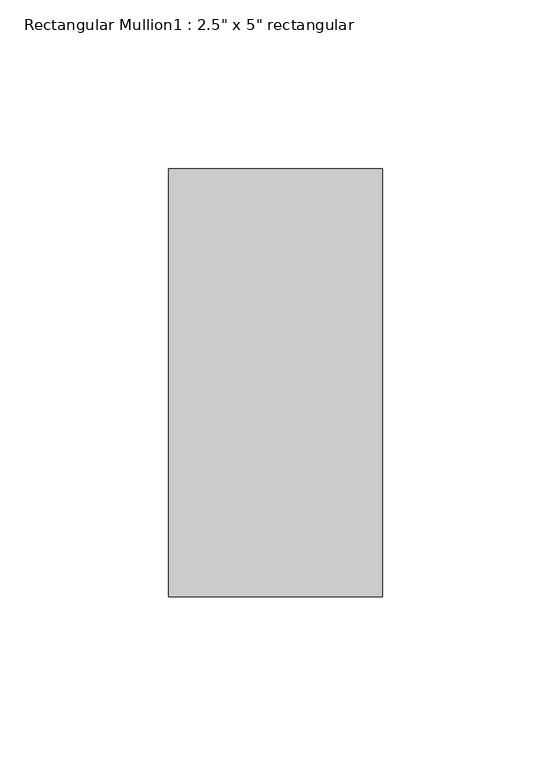
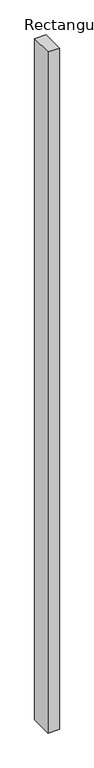
"""IFC4 building model written with IfcOpenShell, lengths in millimetres: member geometry."""

from ifc_helpers import new_model, si_unit, frame, origin, place, context, project, spatial, polyline, outline, extrude, source, transform, mapped, element, save


def member_50cd645d(model_context):
    return source(origin(), model_context, "Body", "SweptSolid", [
        extrude(outline(polyline([(0.0, 63.5), (0.0, -63.5), (-63.5, -63.5), (-63.5, 63.5), (0.0, 63.5)])), frame((0.0, 0.0, -4003.5335741), z_axis=(0.0, 0.0, 1.0), x_axis=(1.0, 0.0, 0.0)), (0.0, 0.0, 1.0), 4003.5335741),
    ])


if __name__ == "__main__":
    model = new_model("IFC4")
    model_context = context("Model", 3, world=origin())
    ifc_project = project(units=[si_unit("LENGTHUNIT", "METRE", prefix="MILLI")], contexts=[model_context])
    site = spatial("IfcSite", under=ifc_project)
    building = spatial("IfcBuilding", under=site)
    placement = place(None, origin())
    member_shape = member_50cd645d(model_context)
    element("IfcMember", 1, ObjectType="Rectangular Mullion1 : 2.5\" x 5\" rectangular", at=placement, inside=building, context=model_context, shape_type="MappedRepresentation", body=[
        mapped(member_shape, transform((0.0, 0.0, 0.0), x_axis=(1.0, 0.0, 0.0), y_axis=(0.0, 1.0, 0.0), z_axis=(0.0, 0.0, 1.0))),
    ])
    save(model, "model.ifc")

# Revit data of these elements
# Type "Rectangular Mullion1 : 2.5\" x 5\" rectangular"
#   built-in parameter 1007304 = 0.416667 (stored number, unit not read)
#   built-in parameter 1007301 = 0.104167 (stored number, unit not read)
#   built-in parameter 1007300 = 0.104167 (stored number, unit not read)
# Element 1 (IfcMember, "Rectangular Mullion1 : 2.5\" x 5\" rectangular")
#   Materials on its faces: "support-frame"
# Materials
#   "support-frame": class "Unassigned", colour RGB 233 233 233, transparency 0, Cost = 0
